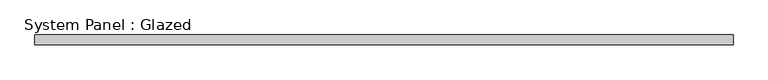
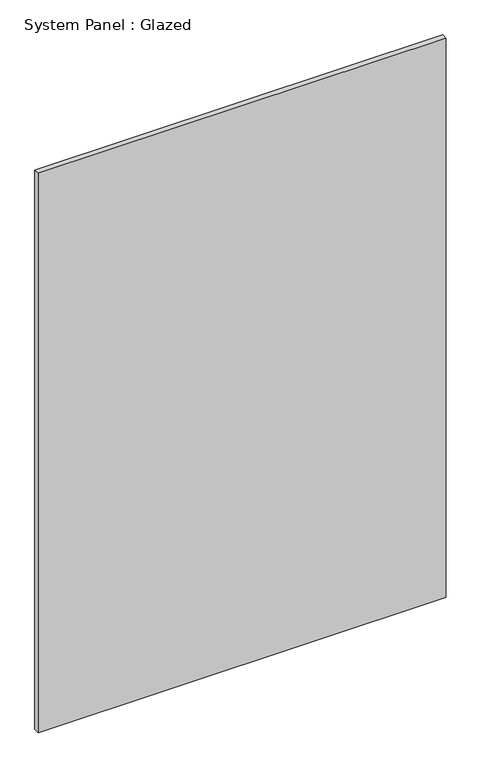
"""IFC4 building model written with IfcOpenShell, lengths in millimetres: plate geometry, System Panel : Glazed."""

from ifc_helpers import new_model, si_unit, origin, origin_with_axes, place, context, project, spatial, polyline, outline, extrude, source, transform, mapped, element, save


def system_panel_glazed_131ccbe9(model_context):
    return source(origin(), model_context, "Body", "SweptSolid", [
        extrude(outline(polyline([(905.5833335, 24.5), (-905.5833335, 24.5), (-905.5833335, 49.5), (905.5833335, 49.5), (905.5833335, 24.5)])), origin_with_axes(), (0.0, 0.0, 1.0), 2625.0),
    ])


if __name__ == "__main__":
    model = new_model("IFC4")
    model_context = context("Model", 3, world=origin())
    ifc_project = project(units=[si_unit("LENGTHUNIT", "METRE", prefix="MILLI")], contexts=[model_context])
    site = spatial("IfcSite", under=ifc_project)
    building = spatial("IfcBuilding", under=site)
    placement = place(None, origin())
    system_panel_glazed_shape = system_panel_glazed_131ccbe9(model_context)
    element("IfcPlate", 1, ObjectType="System Panel : Glazed", at=placement, inside=building, context=model_context, shape_type="MappedRepresentation", body=[
        mapped(system_panel_glazed_shape, transform((0.0, 0.0, 0.0), x_axis=(1.0, 0.0, 0.0), y_axis=(0.0, 1.0, 0.0), z_axis=(0.0, 0.0, 1.0))),
    ])
    save(model, "model.ifc")

# Revit data of these elements
# Element 1 (IfcPlate, "System Panel : Glazed")
#   Materials on its faces: "Glass"
# Materials
#   "Glass": class "Glass", colour RGB 0 128 192, transparency 0.9
